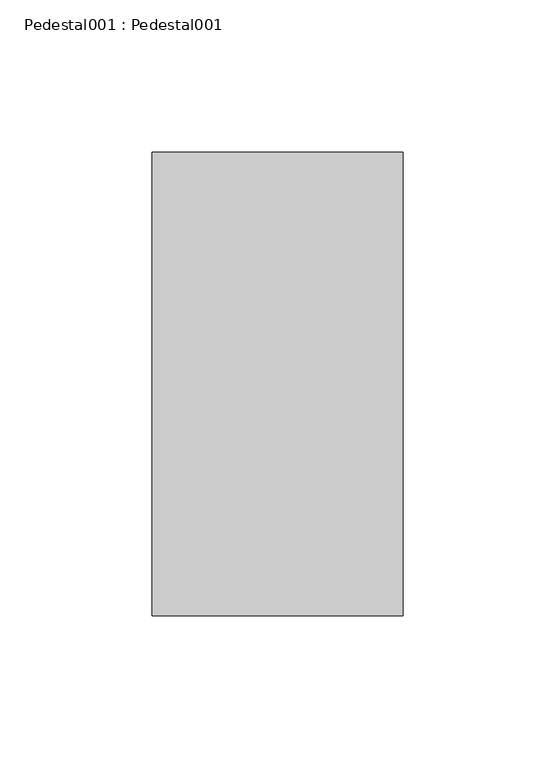
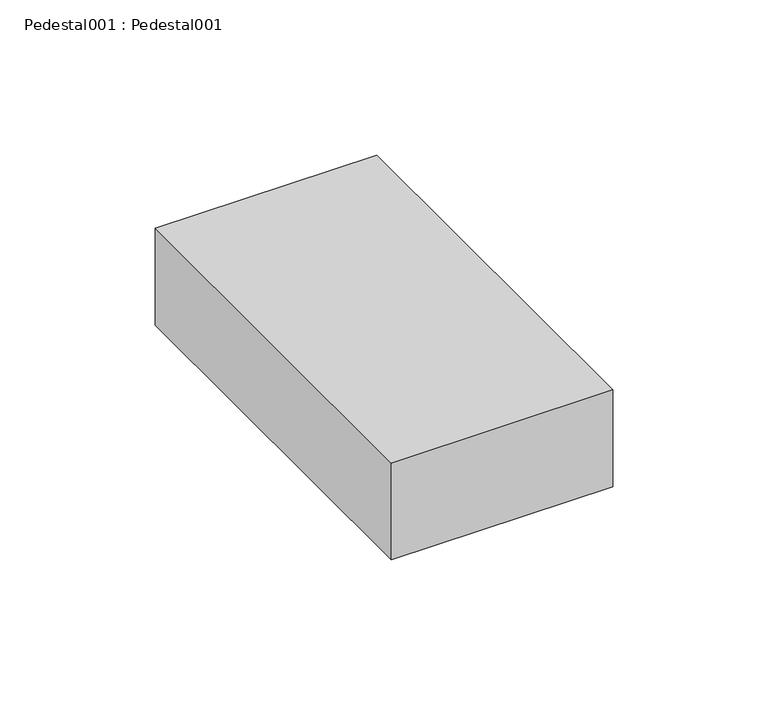
"""IFC4 building model written with IfcOpenShell, lengths in millimetres: proxy geometry, Pedestal001 : Pedestal001."""

from ifc_helpers import new_model, si_unit, frame, origin, place, context, project, spatial, polyline, outline, extrude, source, transform, mapped, element, save


def pedestal001_pedestal001_597e7021(model_context):
    return source(origin(), model_context, "Body", "SweptSolid", [
        extrude(outline(polyline([(-9450.0115234, 9829.7531721), (-9532.5615234, 9829.7531721), (-9532.5615234, 9982.1531721), (-9450.0115234, 9982.1531721), (-9450.0115234, 9829.7531721)])), frame((0.0, 0.0, 40107.9492187), z_axis=(0.0, 0.0, 1.0), x_axis=(1.0, 0.0, 0.0)), (0.0, 0.0, 1.0), 38.1),
    ])


if __name__ == "__main__":
    model = new_model("IFC4")
    model_context = context("Model", 3, world=origin())
    ifc_project = project(units=[si_unit("LENGTHUNIT", "METRE", prefix="MILLI")], contexts=[model_context])
    site = spatial("IfcSite", under=ifc_project)
    building = spatial("IfcBuilding", under=site)
    placement = place(None, origin())
    pedestal001_pedestal001_shape = pedestal001_pedestal001_597e7021(model_context)
    element("IfcBuildingElementProxy", 1, Name="Pedestal001 : Pedestal001", ObjectType="Pedestal001 : Pedestal001", at=placement, inside=building, context=model_context, shape_type="MappedRepresentation", body=[
        mapped(pedestal001_pedestal001_shape, transform((0.0, 0.0, 0.0), x_axis=(1.0, 0.0, 0.0), y_axis=(0.0, 1.0, 0.0), z_axis=(0.0, 0.0, 1.0))),
    ])
    save(model, "model.ifc")

# Revit data of these elements
# Type "Pedestal001 : Pedestal001"
#   NameOverride = "Pedestal001"
# Element 1 (IfcBuildingElementProxy, "Pedestal001 : Pedestal001")
#   Materials on its faces: "BUZON PEDESTAL"
# Materials
#   "BUZON PEDESTAL": class "Unassigned", colour RGB 66 66 66, transparency 0
